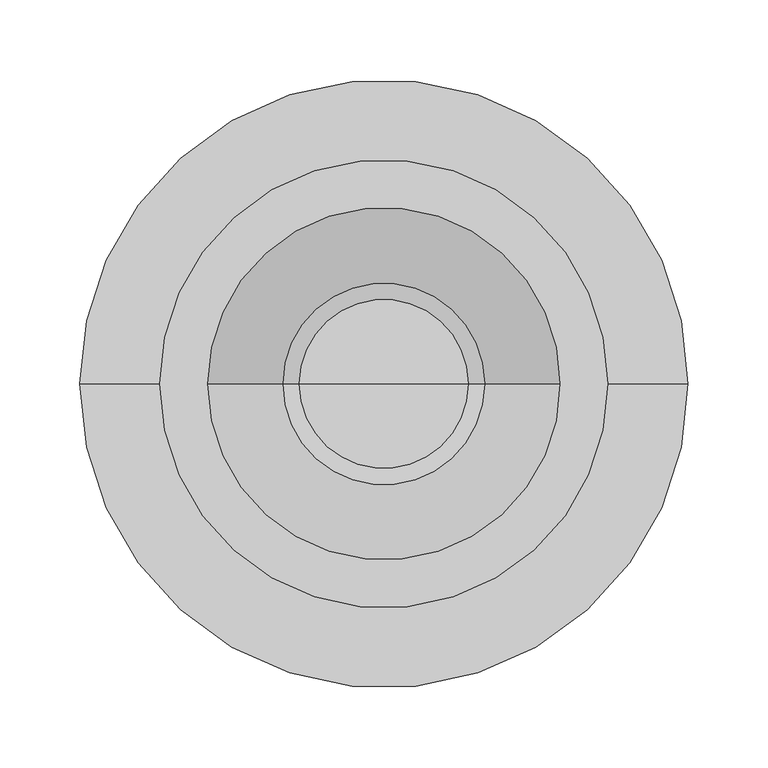
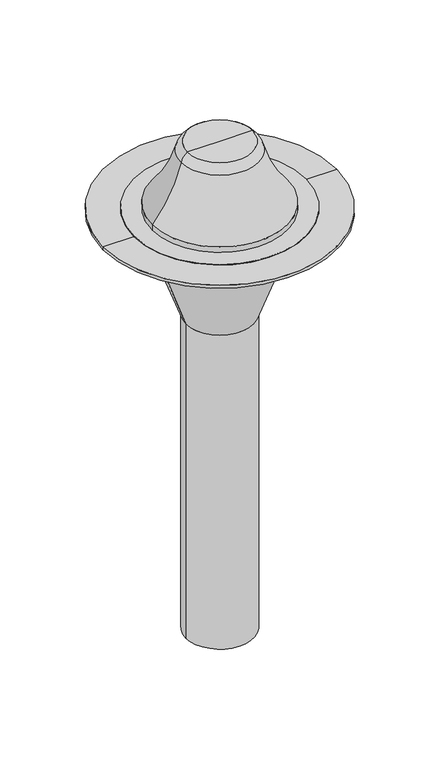
"""IFC4 building model written with IfcOpenShell, lengths in millimetres: proxy geometry, TN_Воронка с обжимным фланцем : Воронка с обжимным металлическим фланцем без обогрева Ø110х720мм."""

from ifc_helpers import new_model, si_unit, point, frame, origin, origin_with_axes, origin_2d, place, context, project, spatial, polyline, circle_curve, ellipse_curve, trimmed, segment, composite_curve, outline, extrude, source, transform, mapped, element, save
from ifc_brep_helpers import plane_surface, cylinder_surface, revolved_surface, advanced_brep


def specialty_equipment_c33bb5df(model_context):
    return source(origin(), model_context, "Body", "SolidModel", [
        advanced_brep(
        [(110.0556416, 0.0, 0.0), (-110.0556416, 0.0, 0.0), (-110.0556416, 0.0, 10.0), (110.0556416, 0.0, 10.0), (0.0, 0.0, 0.0), (52.7728393, 0.0, 115.0), (-52.7728393, 0.0, 115.0), (0.0, 0.0, 115.0), (62.9807579, 0.0, 100.6532382), (-62.9807579, 0.0, 100.6532382)],
        [
            (0, 1, circle_curve(frame((0.0, 0.0, 0.0), z_axis=(0.0, 0.0, 1.0), x_axis=(-1.0, 0.0, 0.0)), 110.0556416)),
            (1, 2),
            (2, 3, circle_curve(frame((0.0, 0.0, 10.0), z_axis=(0.0, 0.0, -1.0), x_axis=(-1.0, 0.0, 0.0)), 110.0556416)),
            (3, 0),
            (1, 0, circle_curve(frame((0.0, 0.0, 0.0), z_axis=(0.0, 0.0, 1.0), x_axis=(-1.0, 0.0, 0.0)), 110.0556416)),
            (3, 2, circle_curve(frame((0.0, 0.0, 10.0), z_axis=(0.0, 0.0, -1.0), x_axis=(-1.0, 0.0, 0.0)), 110.0556416)),
            (4, 1),
            (0, 4),
            (5, 6, circle_curve(frame((0.0, 0.0, 115.0), z_axis=(0.0, 0.0, 1.0), x_axis=(-1.0, 0.0, 0.0)), 52.7728393)),
            (6, 7),
            (7, 5),
            (6, 5, circle_curve(frame((0.0, 0.0, 115.0), z_axis=(0.0, 0.0, 1.0), x_axis=(-1.0, 0.0, 0.0)), 52.7728393)),
            (8, 9, circle_curve(frame((0.0, 0.0, 100.6532382), z_axis=(0.0, 0.0, 1.0), x_axis=(-1.0, 0.0, 0.0)), 62.9807579)),
            (9, 6, circle_curve(frame((-39.8885443, 0.0, 95.0277285), z_axis=(0.0, 1.0, 0.0), x_axis=(1.0, 0.0, 0.0)), 23.7675553)),
            (5, 8, circle_curve(frame((39.8885443, 0.0, 95.0277285), z_axis=(0.0, 1.0, 0.0), x_axis=(-1.0, 0.0, 0.0)), 23.7675553)),
            (9, 8, circle_curve(frame((0.0, 0.0, 100.6532382), z_axis=(0.0, 0.0, 1.0), x_axis=(-1.0, 0.0, 0.0)), 62.9807579)),
            (2, 9, circle_curve(frame((-271.7387744, 0.0, 151.5089197), z_axis=(0.0, -1.0, 0.0), x_axis=(1.0, 0.0, 0.0)), 214.8632351)),
            (8, 3, circle_curve(frame((271.7387744, 0.0, 151.5089197), z_axis=(0.0, -1.0, 0.0), x_axis=(-1.0, 0.0, 0.0)), 214.8632351)),
        ],
        [
            cylinder_surface(frame((0.0, 0.0, 0.0), z_axis=(0.0, 0.0, -1.0), x_axis=(-1.0, 0.0, 0.0)), 110.0556416),
            plane_surface(frame((0.0, 0.0, 0.0), z_axis=(0.0, 0.0, -1.0), x_axis=(-1.0, 0.0, 0.0))),
            plane_surface(frame((0.0, 0.0, 115.0), z_axis=(0.0, 0.0, 1.0), x_axis=(-1.0, 0.0, 0.0))),
            revolved_surface(trimmed(ellipse_curve(frame((-39.8885443, 0.0, 95.0277285), z_axis=(0.0, -1.0, 0.0), x_axis=(1.0, 0.0, 0.0)), 23.7675553, 23.7675553), [point((-52.7728393, 0.0, 115.0))], [point((-62.9807579, 0.0, 100.6532382))], True, "CARTESIAN"), (0.0, 0.0, 0.0), (0.0, 0.0, -1.0)),
            revolved_surface(trimmed(ellipse_curve(frame((-271.7387744, 0.0, 151.5089197), z_axis=(0.0, 1.0, 0.0), x_axis=(1.0, 0.0, 0.0)), 214.8632351, 214.8632351), [point((-62.9807579, 0.0, 100.6532382))], [point((-110.0556416, 0.0, 10.0))], True, "CARTESIAN"), (0.0, 0.0, 0.0), (0.0, 0.0, -1.0)),
        ],
        [
            (0, [[1, 2, 3, 4]]),
            (0, [[5, -4, 6, -2]]),
            (1, [[7, -1, 8]]),
            (1, [[-8, -5, -7]]),
            (2, [[9, 10, 11]]),
            (2, [[12, -11, -10]]),
            (3, [[13, 14, -9, 15]]),
            (3, [[16, -15, -12, -14]]),
            (4, [[-3, 17, -13, 18]]),
            (4, [[-6, -18, -16, -17]]),
        ],
    ),
        extrude(outline(composite_curve([segment(trimmed(circle_curve(origin_2d(), 140.0), [point((-140.0, 0.0))], [point((140.0, 0.0))], False, "CARTESIAN"), True, "CONTINUOUS"), segment(trimmed(circle_curve(origin_2d(), 140.0), [point((140.0, 0.0))], [point((-140.0, 0.0))], False, "CARTESIAN"), True, "CONTINUOUS")], self_intersect=False), holes=[composite_curve([segment(trimmed(circle_curve(origin_2d(), 110.0556416), [point((-110.0556416, 0.0))], [point((110.0556416, 0.0))], True, "CARTESIAN"), True, "CONTINUOUS"), segment(trimmed(circle_curve(origin_2d(), 110.0556416), [point((110.0556416, 0.0))], [point((-110.0556416, 0.0))], True, "CARTESIAN"), True, "CONTINUOUS")], self_intersect=False)]), origin_with_axes(), (0.0, 0.0, 1.0), 1.0),
        advanced_brep(
        [(0.0, 0.0, -720.0), (-55.0, 0.0, -720.0), (55.0, 0.0, -720.0), (190.0, 0.0, 0.0), (-190.0, 0.0, 0.0), (-83.890873, 0.0, 0.0), (83.890873, 0.0, 0.0), (190.0, 0.0, -5.0), (-190.0, 0.0, -5.0), (93.890873, 0.0, -5.0), (-93.890873, 0.0, -5.0), (55.0, 0.0, -179.9935725), (-55.0, 0.0, -179.9935725), (-93.890873, 0.0, -71.109127), (93.890873, 0.0, -71.109127), (81.9669914, 0.0, -74.7632135), (-81.9669914, 0.0, -74.7632135), (0.0, 0.0, -74.7632135), (83.890873, 0.0, -69.3768397), (-83.890873, 0.0, -69.3768397)],
        [
            (0, 1),
            (1, 2, circle_curve(frame((0.0, 0.0, -720.0), z_axis=(0.0, 0.0, -1.0), x_axis=(-1.0, 0.0, 0.0)), 55.0)),
            (2, 0),
            (2, 1, circle_curve(frame((0.0, 0.0, -720.0), z_axis=(0.0, 0.0, -1.0), x_axis=(-1.0, 0.0, 0.0)), 55.0)),
            (3, 4, circle_curve(frame((0.0, 0.0, 0.0), z_axis=(0.0, 0.0, 1.0), x_axis=(-1.0, 0.0, 0.0)), 190.0)),
            (4, 5),
            (5, 6, circle_curve(frame((0.0, 0.0, 0.0), z_axis=(0.0, 0.0, -1.0), x_axis=(-1.0, 0.0, 0.0)), 83.890873)),
            (6, 3),
            (4, 3, circle_curve(frame((0.0, 0.0, 0.0), z_axis=(0.0, 0.0, 1.0), x_axis=(-1.0, 0.0, 0.0)), 190.0)),
            (6, 5, circle_curve(frame((0.0, 0.0, 0.0), z_axis=(0.0, 0.0, -1.0), x_axis=(-1.0, 0.0, 0.0)), 83.890873)),
            (7, 8, circle_curve(frame((0.0, 0.0, -5.0), z_axis=(0.0, 0.0, 1.0), x_axis=(-1.0, 0.0, 0.0)), 190.0)),
            (8, 4),
            (3, 7),
            (8, 7, circle_curve(frame((0.0, 0.0, -5.0), z_axis=(0.0, 0.0, 1.0), x_axis=(-1.0, 0.0, 0.0)), 190.0)),
            (9, 10, circle_curve(frame((0.0, 0.0, -5.0), z_axis=(0.0, 0.0, 1.0), x_axis=(-1.0, 0.0, 0.0)), 93.890873)),
            (10, 8),
            (7, 9),
            (10, 9, circle_curve(frame((0.0, 0.0, -5.0), z_axis=(0.0, 0.0, 1.0), x_axis=(-1.0, 0.0, 0.0)), 93.890873)),
            (11, 12, circle_curve(frame((0.0, 0.0, -179.9935725), z_axis=(0.0, 0.0, 1.0), x_axis=(-1.0, 0.0, 0.0)), 55.0)),
            (12, 13),
            (13, 14, circle_curve(frame((0.0, 0.0, -71.109127), z_axis=(0.0, 0.0, -1.0), x_axis=(-1.0, 0.0, 0.0)), 93.890873)),
            (14, 11),
            (12, 11, circle_curve(frame((0.0, 0.0, -179.9935725), z_axis=(0.0, 0.0, 1.0), x_axis=(-1.0, 0.0, 0.0)), 55.0)),
            (14, 13, circle_curve(frame((0.0, 0.0, -71.109127), z_axis=(0.0, 0.0, -1.0), x_axis=(-1.0, 0.0, 0.0)), 93.890873)),
            (1, 12),
            (11, 2),
            (15, 16, circle_curve(frame((0.0, 0.0, -74.7632135), z_axis=(0.0, 0.0, 1.0), x_axis=(-1.0, 0.0, 0.0)), 81.9669914)),
            (16, 17),
            (17, 15),
            (16, 15, circle_curve(frame((0.0, 0.0, -74.7632135), z_axis=(0.0, 0.0, 1.0), x_axis=(-1.0, 0.0, 0.0)), 81.9669914)),
            (18, 19, circle_curve(frame((0.0, 0.0, -69.3768397), z_axis=(0.0, 0.0, 1.0), x_axis=(-1.0, 0.0, 0.0)), 83.890873)),
            (19, 16),
            (15, 18),
            (19, 18, circle_curve(frame((0.0, 0.0, -69.3768397), z_axis=(0.0, 0.0, 1.0), x_axis=(-1.0, 0.0, 0.0)), 83.890873)),
            (5, 19),
            (18, 6),
            (13, 10),
            (9, 14),
        ],
        [
            plane_surface(frame((0.0, 0.0, -720.0), z_axis=(0.0, 0.0, -1.0), x_axis=(-1.0, 0.0, 0.0))),
            plane_surface(frame((0.0, 0.0, 0.0), z_axis=(0.0, 0.0, 1.0), x_axis=(-1.0, 0.0, 0.0))),
            cylinder_surface(frame((0.0, 0.0, 0.0), z_axis=(0.0, 0.0, -1.0), x_axis=(-1.0, 0.0, 0.0)), 190.0),
            plane_surface(frame((0.0, 0.0, -5.0), z_axis=(0.0, 0.0, -1.0), x_axis=(-1.0, 0.0, 0.0))),
            revolved_surface(polyline([(-93.890873, 0.0, -71.109127), (-55.0, 0.0, -179.9935725)]), (0.0, 0.0, 0.0), (0.0, 0.0, -1.0)),
            cylinder_surface(frame((0.0, 0.0, 0.0), z_axis=(0.0, 0.0, -1.0), x_axis=(-1.0, 0.0, 0.0)), 55.0),
            plane_surface(frame((0.0, 0.0, -74.7632135), z_axis=(0.0, 0.0, 1.0), x_axis=(-1.0, 0.0, 0.0))),
            revolved_surface(polyline([(-81.9669914, 0.0, -74.7632135), (-83.890873, 0.0, -69.3768397)]), (0.0, 0.0, 0.0), (0.0, 0.0, -1.0)),
            revolved_surface(polyline([(-83.890873, 0.0, -69.3768397), (-83.890873, 0.0, 0.0)]), (0.0, 0.0, 0.0), (0.0, 0.0, -1.0)),
            cylinder_surface(frame((0.0, 0.0, 0.0), z_axis=(0.0, 0.0, -1.0), x_axis=(-1.0, 0.0, 0.0)), 93.890873),
        ],
        [
            (0, [[1, 2, 3]]),
            (0, [[-3, 4, -1]]),
            (1, [[5, 6, 7, 8]]),
            (1, [[9, -8, 10, -6]]),
            (2, [[11, 12, -5, 13]]),
            (2, [[14, -13, -9, -12]]),
            (3, [[15, 16, -11, 17]]),
            (3, [[18, -17, -14, -16]]),
            (4, [[19, 20, 21, 22]]),
            (4, [[23, -22, 24, -20]]),
            (5, [[-2, 25, -19, 26]]),
            (5, [[-4, -26, -23, -25]]),
            (6, [[27, 28, 29]]),
            (6, [[30, -29, -28]]),
            (7, [[31, 32, -27, 33]]),
            (7, [[34, -33, -30, -32]]),
            (8, [[-7, 35, -31, 36]]),
            (8, [[-10, -36, -34, -35]]),
            (9, [[-21, 37, -15, 38]]),
            (9, [[-24, -38, -18, -37]]),
        ],
    ),
    ])


if __name__ == "__main__":
    model = new_model("IFC4")
    model_context = context("Model", 3, world=origin())
    ifc_project = project(units=[si_unit("LENGTHUNIT", "METRE", prefix="MILLI")], contexts=[model_context])
    site = spatial("IfcSite", under=ifc_project)
    building = spatial("IfcBuilding", under=site)
    placement = place(None, origin())
    specialty_equipment_shape = specialty_equipment_c33bb5df(model_context)
    element("IfcBuildingElementProxy", 1, Name="TN_Воронка с обжимным фланцем : Воронка с обжимным металлическим фланцем без обогрева Ø110х720мм", ObjectType="TN_Воронка с обжимным фланцем : Воронка с обжимным металлическим фланцем без обогрева Ø110х720мм", at=placement, inside=building, context=model_context, shape_type="MappedRepresentation", body=[
        mapped(specialty_equipment_shape, transform((0.0, 0.0, 0.0), x_axis=(1.0, 0.0, 0.0), y_axis=(0.0, 1.0, 0.0), z_axis=(0.0, 0.0, 1.0))),
    ])
    save(model, "model.ifc")

# Revit data of these elements
# Type "TN_Воронка с обжимным фланцем : Воронка с обжимным металлическим фланцем без обогрева Ø110х720мм"
#   ADSK_Группирование = "Комплектующие и воронки"
#   Description = "Кровельная воронка ТЕХНОНИКОЛЬ является универсальным средством для отвода воды с поверхности плоских кровель, в устройстве которых использовались ПВХ и ТПО мембраны. Для более эффективной работы воронка оснащена листоуловителем, а для простоты монтажа – обжимным фланцем.\r\n\r\nИспользовать воронку можно во всех климатических регионах, т.к. она не плавится при температуре до +70 С и не становится ломкой до – 55 С. Дополнительно для защиты от солнца в состав добавлены УФ-стабилизаторы, обеспечивающие устойчивость к ультрафиолетовому и атмосферному воздействию в диапазоне температур от минус 50 до плюс 90 °С.\r\n\r\nБлагодаря механическому способу крепления, воронка подходит для всех типов полимерных кровельных материалов. Воронка крепится с помощью гаек и барашков, либо пластиковым закручивающимся фланцем. В комплект входит гайки, барашки, а также инструмент для затягивания пластикового фланца."
#   Manufacturer = "ТехноНИКОЛЬ"
#   URL = "https://shop.tn.ru/voronka-s-obzhimnym-metallicheskim-flancem-bez-obogreva-o110h720mm"
#   ADSK_Примечание = ""
#   ADSK_Обозначение = "ТехноНИКОЛЬ"
#   ADSK_Наименование = "Воронка с обжимным металлическим фланцем без обогрева Ø110х720мм"
#   ADSK_Масса_Текст = ""
#   ADSK_Марка = ""
#   ADSK_Код изделия = "671702"
#   ADSK_Завод-изготовитель = "ТехноНИКОЛЬ"
#   ADSK_Единица измерения = "шт."
#   ADSK_Группирование = "Комплектующие и воронки"
#   ADSK_URL страницы изделия = "https://shop.tn.ru/voronka-s-obzhimnym-metallicheskim-flancem-bez-obogreva-o110h720mm"
#   ADSK_URL документации изделия = "https://shop.tn.ru/media/other_documents/_661125_661124_661134_671701_671702_661132_661131_661130_4.pdf"
#   Тип воронки = 2
#   Радиус = 55 mm
#   Пропускная способность = 7.8 L/s
#   Монтажный диаметр = 110 mm
#   Длина расчетная [instance default] = 720 mm
#   Длина отвода [instance default] = 720 mm
#   ADSK_Масса = 2
#   ADSK_Количество = 1
#   Видимость_Листоуловитель [instance default] = yes
#   Материал_Фланец = TN_ПВХ_Серый
#   Материал_Корпус = TN_ПВХ_Черный
#   Default Elevation = 0
# Element 1 (IfcBuildingElementProxy, "TN_Воронка с обжимным фланцем : Воронка с обжимным металлическим фланцем без обогрева Ø110х720мм")
#   Materials on its faces: "TN_ПВХ_Черный", "TN_ПВХ_Серый"
# Materials
#   "TN_ПВХ_Серый": class "Типовые", colour RGB 192 192 192, transparency 0, Cost = 0
#   "TN_ПВХ_Черный": class "Типовые", colour RGB 48 48 48, transparency 0, Cost = 0
